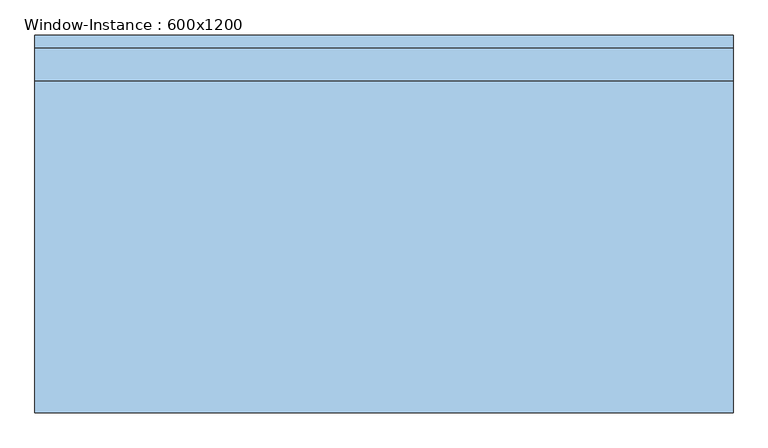
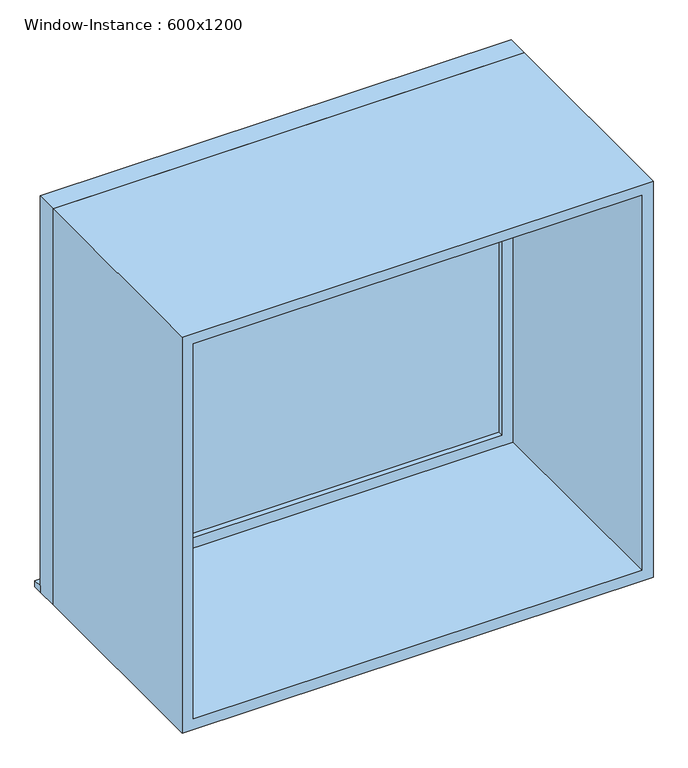
"""IFC4 building model written with IfcOpenShell, lengths in millimetres: window geometry, Window-Instance : 600x1200."""

from ifc_helpers import new_model, si_unit, frame, origin, place, context, project, spatial, polyline, outline, extrude, source, transform, mapped, element, save


def window_instance_600x1200_a5f13d3b(model_context):
    return source(origin(), model_context, "Body", "SweptSolid", [
        extrude(outline(polyline([(-713.1, 377.9), (636.9, 377.9), (636.9, 352.5), (-713.1, 352.5), (-713.1, 377.9)])), frame((0.0, 0.0, 900.0), z_axis=(0.0, 0.0, 1.0), x_axis=(1.0, 0.0, 0.0)), (0.0, 0.0, 1.0), 19.05),
        extrude(outline(polyline([(573.4, 303.925), (-649.6, 303.925), (-649.6, 316.625), (573.4, 316.625), (573.4, 303.925)])), frame((0.0, 0.0, 963.5), z_axis=(0.0, 0.0, 1.0), x_axis=(1.0, 0.0, 0.0)), (0.0, 0.0, 1.0), 1073.0),
        extrude(outline(polyline([(2080.95, -694.05), (919.05, -694.05), (919.05, 617.85), (2080.95, 617.85), (2080.95, -694.05)]), holes=[polyline([(2036.5, -649.6), (2036.5, 573.4), (963.5, 573.4), (963.5, -649.6), (2036.5, -649.6)])]), frame((0.0, 288.05, 0.0), z_axis=(0.0, 1.0, 0.0), x_axis=(0.0, 0.0, 1.0)), (0.0, 0.0, 1.0), 44.45),
        extrude(outline(polyline([(2100.0, -713.1), (900.0, -713.1), (900.0, 636.9), (2100.0, 636.9), (2100.0, -713.1)]), holes=[polyline([(2068.25, -681.35), (2068.25, 605.15), (931.75, 605.15), (931.75, -681.35), (2068.25, -681.35)])]), frame((0.0, -352.5, 0.0), z_axis=(0.0, 1.0, 0.0), x_axis=(0.0, 0.0, 1.0)), (0.0, 0.0, 1.0), 640.55),
        extrude(outline(polyline([(2100.0, 636.9), (2100.0, -713.1), (900.0, -713.1), (900.0, 636.9), (2100.0, 636.9)]), holes=[polyline([(2080.95, 617.85), (919.05, 617.85), (919.05, -694.05), (2080.95, -694.05), (2080.95, 617.85)])]), frame((0.0, 288.05, 0.0), z_axis=(0.0, 1.0, 0.0), x_axis=(0.0, 0.0, 1.0)), (0.0, 0.0, 1.0), 64.45),
    ])


if __name__ == "__main__":
    model = new_model("IFC4")
    model_context = context("Model", 3, world=origin())
    ifc_project = project(units=[si_unit("LENGTHUNIT", "METRE", prefix="MILLI")], contexts=[model_context])
    site = spatial("IfcSite", under=ifc_project)
    building = spatial("IfcBuilding", under=site)
    placement = place(None, origin())
    window_instance_600x1200_shape = window_instance_600x1200_a5f13d3b(model_context)
    element("IfcWindow", 1, ObjectType="Window-Instance : 600x1200", at=placement, inside=building, context=model_context, shape_type="MappedRepresentation", body=[
        mapped(window_instance_600x1200_shape, transform((0.0, 0.0, 0.0), x_axis=(1.0, 0.0, 0.0), y_axis=(0.0, 1.0, 0.0), z_axis=(0.0, 0.0, 1.0))),
    ])
    save(model, "model.ifc")

# Revit data of these elements
# Type "Window-Instance : 600x1200"
#   Type Mark = "7"
#   Construction Type Id = "GSP4R"
#   Assembly Code = "B2020100"
#   Analytic Construction = "1/8 in Pilkington single glazing"
#   Visual Light Transmittance = 0.9
#   Thermal Resistance (R) = 0.149095 (m²·K)/W
#   Solar Heat Gain Coefficient = 0.86
#   Heat Transfer Coefficient (U) = 6.70716 W/(m²·K)
#   Height [instance default] = 1200 mm
#   Default Sill Height = 900 mm
#   Width [instance default] = 600 mm
#   Window Inset = 20 mm
#   Glass Pane Material = WW-EC-GL-Storefront
#   Sash Material = WW-EC-RGB-White
#   Wall Closure = (empty or 0)
# Element 1 (IfcWindow, "Window-Instance : 600x1200")
#   Width = 1350 mm
#   Materials on its faces: "WW-EC-RGB-White", "WW-EC-GL-Storefront"
# Materials
#   "WW-EC-GL-Storefront": class "Glass", colour RGB 236 240 239, transparency 0.85, Description = "Storefront Glass", Cost = 0
#   "WW-EC-RGB-White": class "Generic", colour RGB 255 255 255, transparency 0, Comments = "If region requests off-white, swith asset color to RGB 231-228-220", Description = "Generic Color", Cost = 0
